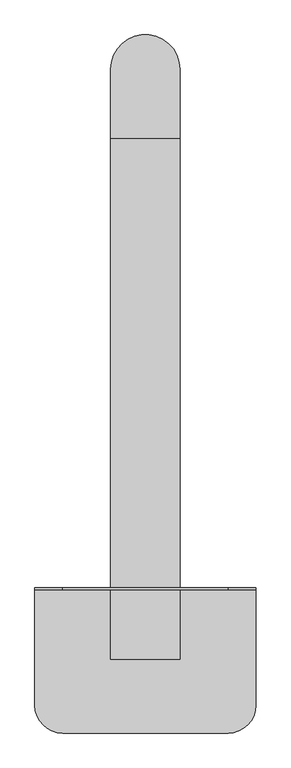
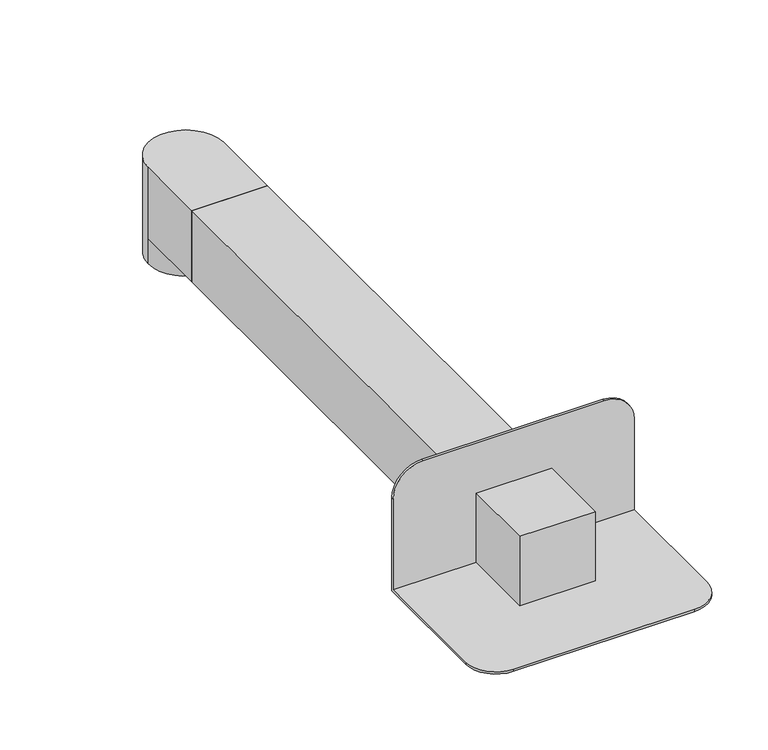
"""IFC4 building model written with IfcOpenShell, lengths in millimetres: proxy geometry, TN_ПВХ воронка парапетная : ПВХ воронка парапетная 100х100 длиной 650мм с отводом и листоуловителем."""

from ifc_helpers import new_model, si_unit, frame, origin, place, context, project, spatial, polyline, circle_curve, outline, extrude, source, transform, mapped, element, save
from ifc_brep_helpers import plane_surface, cylinder_surface, revolved_surface, advanced_brep


def specialty_equipment_25f16bf1(model_context):
    return source(origin(), model_context, "Body", "SolidModel", [
        extrude(outline(polyline([(50.0, -3.286311), (50.0, -103.286311), (-50.0, -103.286311), (-50.0, -3.286311), (50.0, -3.286311)])), frame((0.0, 0.0, 3.0), z_axis=(0.0, 0.0, 1.0), x_axis=(1.0, 0.0, 0.0)), (0.0, 0.0, 1.0), 97.0),
        advanced_brep(
        [(-47.0, 750.0, 97.0), (47.0, 750.0, 97.0), (47.0, 750.0, -35.0), (-47.0, 750.0, -35.0), (50.0, 650.0, 0.0), (50.0, 650.0, 100.0), (-50.0, 650.0, 100.0), (-50.0, 650.0, 0.0), (47.0, 650.0, 3.0), (-47.0, 650.0, 3.0), (-47.0, 650.0, 97.0), (47.0, 650.0, 97.0), (50.0, 750.0, 0.0), (50.0, 750.0, 100.0), (-50.0, 750.0, 100.0), (-50.0, 750.0, 0.0), (47.0, 732.9412779, 3.0), (-47.0, 732.9412779, 3.0), (-47.0, 732.9412779, 97.0), (47.0, 732.9412779, 97.0), (-50.0, 750.0, -35.0), (50.0, 750.0, -35.0)],
        [
            (0, 1, circle_curve(frame((0.0, 750.0, 97.0), z_axis=(0.0, 0.0, -1.0), x_axis=(1.0, 0.0, 0.0)), 47.0)),
            (1, 0, circle_curve(frame((0.0, 750.0, 97.0), z_axis=(0.0, 0.0, -1.0), x_axis=(1.0, 0.0, 0.0)), 47.0)),
            (1, 2),
            (2, 3, circle_curve(frame((0.0, 750.0, -35.0), z_axis=(0.0, 0.0, -1.0), x_axis=(1.0, 0.0, 0.0)), 47.0)),
            (3, 0),
            (3, 2, circle_curve(frame((0.0, 750.0, -35.0), z_axis=(0.0, 0.0, -1.0), x_axis=(1.0, 0.0, 0.0)), 47.0)),
            (4, 5),
            (5, 6),
            (6, 7),
            (7, 4),
            (8, 9),
            (9, 10),
            (10, 11),
            (11, 8),
            (4, 12),
            (12, 13),
            (13, 5),
            (13, 14, circle_curve(frame((0.0, 750.0, 100.0), z_axis=(0.0, 0.0, 1.0), x_axis=(1.0, 0.0, 0.0)), 50.0)),
            (14, 6),
            (14, 15),
            (15, 7),
            (15, 12, circle_curve(frame((0.0, 750.0, 0.0), z_axis=(0.0, 0.0, 1.0), x_axis=(1.0, 0.0, 0.0)), 50.0)),
            (8, 16),
            (16, 17, circle_curve(frame((0.0, 750.0, 3.0), z_axis=(0.0, 0.0, -1.0), x_axis=(1.0, 0.0, 0.0)), 50.0)),
            (17, 9),
            (17, 18),
            (18, 10),
            (18, 19, circle_curve(frame((0.0, 750.0, 97.0), z_axis=(0.0, 0.0, 1.0), x_axis=(1.0, 0.0, 0.0)), 50.0)),
            (19, 11),
            (19, 16),
            (20, 21, circle_curve(frame((0.0, 750.0, -35.0), z_axis=(0.0, 0.0, -1.0), x_axis=(1.0, 0.0, 0.0)), 50.0)),
            (21, 20, circle_curve(frame((0.0, 750.0, -35.0), z_axis=(0.0, 0.0, -1.0), x_axis=(1.0, 0.0, 0.0)), 50.0)),
            (21, 12),
            (15, 20),
        ],
        [
            plane_surface(frame((47.0, 750.0, 97.0), z_axis=(0.0, 0.0, -1.0), x_axis=(0.0, 1.0, 0.0))),
            revolved_surface(polyline([(47.0, 750.0, 97.0), (47.0, 750.0, -35.0)]), (0.0, 750.0, -35.0), (0.0, 0.0, 1.0)),
            plane_surface(frame((-50.0, 650.0, 0.0), z_axis=(0.0, -1.0, 0.0), x_axis=(1.0, 0.0, 0.0))),
            plane_surface(frame((50.0, 750.0, 100.0), z_axis=(1.0, 0.0, 0.0), x_axis=(0.0, -1.0, 0.0))),
            plane_surface(frame((-50.0, 750.0, 100.0), z_axis=(0.0, 0.0, 1.0), x_axis=(0.0, -1.0, 0.0))),
            plane_surface(frame((-50.0, 750.0, 0.0), z_axis=(-1.0, 0.0, 0.0), x_axis=(0.0, -1.0, 0.0))),
            plane_surface(frame((50.0, 750.0, 0.0), z_axis=(0.0, 0.0, -1.0), x_axis=(0.0, -1.0, 0.0))),
            plane_surface(frame((-47.0, 750.0, 3.0), z_axis=(0.0, 0.0, 1.0), x_axis=(0.0, -1.0, 0.0))),
            plane_surface(frame((-47.0, 750.0, 97.0), z_axis=(1.0, 0.0, 0.0), x_axis=(0.0, -1.0, 0.0))),
            plane_surface(frame((47.0, 750.0, 97.0), z_axis=(0.0, 0.0, -1.0), x_axis=(0.0, -1.0, 0.0))),
            plane_surface(frame((47.0, 750.0, 3.0), z_axis=(-1.0, 0.0, 0.0), x_axis=(0.0, -1.0, 0.0))),
            plane_surface(frame((50.0, 750.0, -35.0), z_axis=(0.0, 0.0, -1.0), x_axis=(0.0, -1.0, 0.0))),
            cylinder_surface(frame((0.0, 750.0, -35.0), z_axis=(0.0, 0.0, 1.0), x_axis=(1.0, 0.0, 0.0)), 50.0),
        ],
        [
            (0, [[1, 2]]),
            (1, [[-2, 3, 4, 5]]),
            (1, [[-1, -5, 6, -3]]),
            (2, [[7, 8, 9, 10], [11, 12, 13, 14]]),
            (3, [[-7, 15, 16, 17]]),
            (4, [[-8, -17, 18, 19]]),
            (5, [[-9, -19, 20, 21]]),
            (6, [[-10, -21, 22, -15]]),
            (7, [[-11, 23, 24, 25]]),
            (8, [[-12, -25, 26, 27]]),
            (9, [[-13, -27, 28, 29]]),
            (10, [[-14, -29, 30, -23]]),
            (11, [[31, 32], [-4, -6]]),
            (12, [[-24, -30, -28, -26]]),
            (12, [[-32, 33, -22, 34]]),
            (12, [[-18, -16, -33, -31, -34, -20]]),
        ],
    ),
        advanced_brep(
        [(50.0, 650.0, 0.0), (-50.0, 650.0, 0.0), (-50.0, 650.0, 100.0), (50.0, 650.0, 100.0), (47.0, 650.0, 3.0), (47.0, 650.0, 97.0), (-47.0, 650.0, 97.0), (-47.0, 650.0, 3.0), (50.0, 0.0, 100.0), (50.0, 0.0, 0.0), (-50.0, 0.0, 100.0), (-50.0, 0.0, 0.0), (160.0, 0.0, 0.0), (160.0, -170.0, 0.0), (120.0, -210.0, 0.0), (-120.0, -210.0, 0.0), (-160.0, -170.0, 0.0), (-160.0, 0.0, 0.0), (-47.0, -3.0, 3.0), (-160.0, -3.0, 3.0), (-160.0, -170.0, 3.0), (-120.0, -210.0, 3.0), (120.0, -210.0, 3.0), (160.0, -170.0, 3.0), (160.0, -3.0, 3.0), (47.0, -3.0, 3.0), (-47.0, -3.0, 97.0), (47.0, -3.0, 97.0), (160.0, -3.0, 130.0), (120.0, -3.0, 170.0), (-120.0, -3.0, 170.0), (-160.0, -3.0, 130.0), (-160.0, 0.0, 130.0), (-120.0, 0.0, 170.0), (120.0, 0.0, 170.0), (160.0, 0.0, 130.0)],
        [
            (0, 1),
            (1, 2),
            (2, 3),
            (3, 0),
            (4, 5),
            (5, 6),
            (6, 7),
            (7, 4),
            (3, 8),
            (8, 9),
            (9, 0),
            (2, 10),
            (10, 8),
            (1, 11),
            (11, 10),
            (9, 12),
            (12, 13),
            (13, 14, circle_curve(frame((120.0, -170.0, 0.0), z_axis=(0.0, 0.0, -1.0), x_axis=(1.0, 0.0, 0.0)), 40.0)),
            (14, 15),
            (15, 16, circle_curve(frame((-120.0, -170.0, 0.0), z_axis=(0.0, 0.0, -1.0), x_axis=(1.0, 0.0, 0.0)), 40.0)),
            (16, 17),
            (17, 11),
            (7, 18),
            (18, 19),
            (19, 20),
            (20, 21, circle_curve(frame((-120.0, -170.0, 3.0), z_axis=(0.0, 0.0, 1.0), x_axis=(1.0, 0.0, 0.0)), 40.0)),
            (21, 22),
            (22, 23, circle_curve(frame((120.0, -170.0, 3.0), z_axis=(0.0, 0.0, 1.0), x_axis=(1.0, 0.0, 0.0)), 40.0)),
            (23, 24),
            (24, 25),
            (25, 4),
            (6, 26),
            (26, 18),
            (5, 27),
            (27, 26),
            (25, 27),
            (24, 28),
            (28, 29, circle_curve(frame((120.0, -3.0, 130.0), z_axis=(0.0, -1.0, 0.0), x_axis=(1.0, 0.0, 0.0)), 40.0)),
            (29, 30),
            (30, 31, circle_curve(frame((-120.0, -3.0, 130.0), z_axis=(0.0, -1.0, 0.0), x_axis=(1.0, 0.0, 0.0)), 40.0)),
            (31, 19),
            (32, 33, circle_curve(frame((-120.0, 0.0, 130.0), z_axis=(0.0, 1.0, 0.0), x_axis=(1.0, 0.0, 0.0)), 40.0)),
            (33, 34),
            (34, 35, circle_curve(frame((120.0, 0.0, 130.0), z_axis=(0.0, 1.0, 0.0), x_axis=(1.0, 0.0, 0.0)), 40.0)),
            (35, 12),
            (17, 32),
            (23, 13),
            (35, 28),
            (34, 29),
            (33, 30),
            (32, 31),
            (16, 20),
            (15, 21),
            (14, 22),
        ],
        [
            plane_surface(frame((50.0, 650.0, 0.0), z_axis=(0.0, 1.0, 0.0), x_axis=(0.0, 0.0, -1.0))),
            plane_surface(frame((50.0, 0.0, 0.0), z_axis=(1.0, 0.0, 0.0), x_axis=(0.0, 1.0, 0.0))),
            plane_surface(frame((50.0, 0.0, 100.0), z_axis=(0.0, 0.0, 1.0), x_axis=(0.0, 1.0, 0.0))),
            plane_surface(frame((-50.0, 0.0, 100.0), z_axis=(-1.0, 0.0, 0.0), x_axis=(0.0, 1.0, 0.0))),
            plane_surface(frame((-50.0, 0.0, 0.0), z_axis=(0.0, 0.0, -1.0), x_axis=(0.0, 1.0, 0.0))),
            plane_surface(frame((47.0, 0.0, 3.0), z_axis=(0.0, 0.0, 1.0), x_axis=(0.0, 1.0, 0.0))),
            plane_surface(frame((-47.0, 0.0, 3.0), z_axis=(1.0, 0.0, 0.0), x_axis=(0.0, 1.0, 0.0))),
            plane_surface(frame((-47.0, 0.0, 97.0), z_axis=(0.0, 0.0, -1.0), x_axis=(0.0, 1.0, 0.0))),
            plane_surface(frame((47.0, 0.0, 97.0), z_axis=(-1.0, 0.0, 0.0), x_axis=(0.0, 1.0, 0.0))),
            plane_surface(frame((160.0, -3.0, 130.0), z_axis=(0.0, -1.0, 0.0), x_axis=(0.0, 0.0, 1.0))),
            plane_surface(frame((160.0, 0.0, 130.0), z_axis=(0.0, 1.0, 0.0), x_axis=(0.0, 0.0, -1.0))),
            plane_surface(frame((160.0, -3.0, 3.0), z_axis=(1.0, 0.0, 0.0), x_axis=(0.0, 1.0, 0.0))),
            cylinder_surface(frame((120.0, 0.0, 130.0), z_axis=(0.0, -1.0, 0.0), x_axis=(1.0, 0.0, 0.0)), 40.0),
            plane_surface(frame((120.0, -3.0, 170.0), z_axis=(0.0, 0.0, 1.0), x_axis=(0.0, 1.0, 0.0))),
            cylinder_surface(frame((-120.0, 0.0, 130.0), z_axis=(0.0, -1.0, 0.0), x_axis=(1.0, 0.0, 0.0)), 40.0),
            plane_surface(frame((-160.0, -3.0, 130.0), z_axis=(-1.0, 0.0, 0.0), x_axis=(0.0, 1.0, 0.0))),
            cylinder_surface(frame((-120.0, -170.0, 0.0), z_axis=(0.0, 0.0, 1.0), x_axis=(1.0, 0.0, 0.0)), 40.0),
            plane_surface(frame((-120.0, -210.0, 3.0), z_axis=(0.0, -1.0, 0.0), x_axis=(0.0, 0.0, -1.0))),
            cylinder_surface(frame((120.0, -170.0, 0.0), z_axis=(0.0, 0.0, 1.0), x_axis=(1.0, 0.0, 0.0)), 40.0),
        ],
        [
            (0, [[1, 2, 3, 4], [5, 6, 7, 8]]),
            (1, [[-4, 9, 10, 11]]),
            (2, [[-3, 12, 13, -9]]),
            (3, [[-2, 14, 15, -12]]),
            (4, [[-1, -11, 16, 17, 18, 19, 20, 21, 22, -14]]),
            (5, [[-8, 23, 24, 25, 26, 27, 28, 29, 30, 31]]),
            (6, [[-23, -7, 32, 33]]),
            (7, [[-6, 34, 35, -32]]),
            (8, [[-5, -31, 36, -34]]),
            (9, [[37, 38, 39, 40, 41, -24, -33, -35, -36, -30]]),
            (10, [[42, 43, 44, 45, -16, -10, -13, -15, -22, 46]]),
            (11, [[-37, -29, 47, -17, -45, 48]]),
            (12, [[-38, -48, -44, 49]]),
            (13, [[-39, -49, -43, 50]]),
            (14, [[-40, -50, -42, 51]]),
            (15, [[-41, -51, -46, -21, 52, -25]]),
            (16, [[-26, -52, -20, 53]]),
            (17, [[-27, -53, -19, 54]]),
            (18, [[-28, -54, -18, -47]]),
        ],
    ),
    ])


if __name__ == "__main__":
    model = new_model("IFC4")
    model_context = context("Model", 3, world=origin())
    ifc_project = project(units=[si_unit("LENGTHUNIT", "METRE", prefix="MILLI")], contexts=[model_context])
    site = spatial("IfcSite", under=ifc_project)
    building = spatial("IfcBuilding", under=site)
    placement = place(None, origin())
    specialty_equipment_shape = specialty_equipment_25f16bf1(model_context)
    element("IfcBuildingElementProxy", 1, Name="TN_ПВХ воронка парапетная : ПВХ воронка парапетная 100х100 длиной 650мм с отводом и листоуловителем", ObjectType="TN_ПВХ воронка парапетная : ПВХ воронка парапетная 100х100 длиной 650мм с отводом и листоуловителем", at=placement, inside=building, context=model_context, shape_type="MappedRepresentation", body=[
        mapped(specialty_equipment_shape, transform((0.0, 0.0, 0.0), x_axis=(1.0, 0.0, 0.0), y_axis=(0.0, 1.0, 0.0), z_axis=(0.0, 0.0, 1.0))),
    ])
    save(model, "model.ifc")

# Revit data of these elements
# Type "TN_ПВХ воронка парапетная : ПВХ воронка парапетная 100х100 длиной 650мм с отводом и листоуловителем"
#   ADSK_Группирование = "Комплектующие и воронки"
#   Description = "ПВХ воронка парапетная 100х100 длиной 650мм с отводом и листоуловителем  применяется для организации внешнего водостока через балконы и парапеты на пониженных участках кровли."
#   Manufacturer = "ТехноНИКОЛЬ"
#   URL = "https://tnsystem.ru/pvkh-voronka-parapetnaya-100kh100-dlinoy-650mm-s-otvodom-i-listoulovitelem/"
#   ADSK_Примечание = ""
#   ADSK_Обозначение = "ТехноНИКОЛЬ"
#   ADSK_Наименование = "ПВХ воронка парапетная 100х100 длиной 650мм с отводом и листоуловителем"
#   ADSK_Марка = ""
#   ADSK_Код изделия = "693437"
#   ADSK_Завод-изготовитель = "ТехноНИКОЛЬ"
#   ADSK_Единица измерения = "шт."
#   ADSK_Группирование = "Комплектующие и воронки"
#   ADSK_URL страницы изделия = "https://tnsystem.ru/pvkh-voronka-parapetnaya-100kh100-dlinoy-650mm-s-otvodom-i-listoulovitelem/"
#   ADSK_URL документации изделия = "https://logicroof.ru/upload/iblock/83e/83e7fce9cad6548c00142fa93d3ba2c3.pdf"
#   Тип воронки = 3
#   Длина расчетная [instance default] = 650 mm
#   Длина отвода [instance default] = 650 mm
#   ADSK_Размер_Ширина = 100 mm
#   ADSK_Размер_Высота = 100 mm
#   ADSK_Количество = 1
#   Видимость_Переход [instance default] = yes
#   Видимость_Листоуловитель [instance default] = yes
#   Видимость отвода [instance default] = yes
#   Видимость листоуловителя [instance default] = yes
#   Материал_Листоуловитель = TN_ПВХ_Черный
#   Материал_Корпус = TN_ПВХ_Серый
#   Default Elevation = 0
# Element 1 (IfcBuildingElementProxy, "TN_ПВХ воронка парапетная : ПВХ воронка парапетная 100х100 длиной 650мм с отводом и листоуловителем")
#   Materials on its faces: "TN_ПВХ_Серый", "TN_ПВХ_Черный"
# Materials
#   "TN_ПВХ_Черный": class "Типовые", colour RGB 48 48 48, transparency 0, Cost = 0
#   "TN_ПВХ_Серый": class "Типовые", colour RGB 192 192 192, transparency 0, Cost = 0
